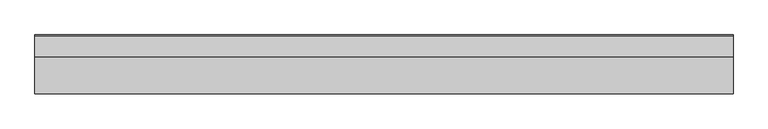
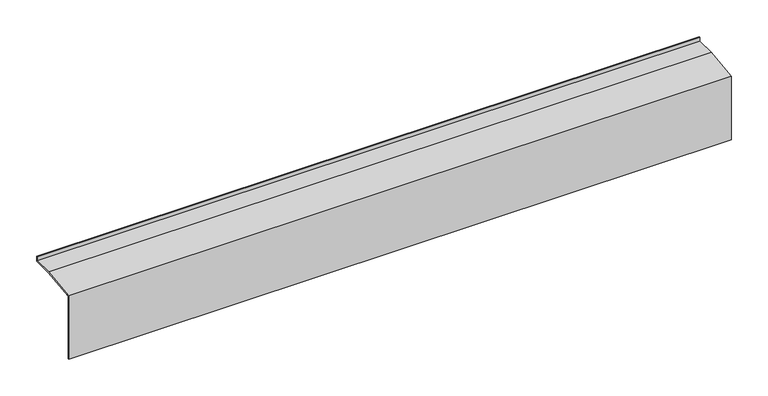
"""IFC4 building model written with IfcOpenShell, lengths in millimetres: proxy geometry, Generic Models 7:Generic Models 1:7:Generic Models 1:7 : Generic Models 7:Generic Models 1:337419:2 : Generic Models 7:Generic Models 1:7:Generic Models 1:7 : Generic Models 7:Generic Models 1:337419:315055."""

from ifc_helpers import new_model, si_unit, frame, origin, place, context, project, spatial, polyline, outline, extrude, source, transform, mapped, element, save


def generic_models_7c3e0f65(model_context):
    return source(origin(), model_context, "Body", "SweptSolid", [
        extrude(outline(polyline([(-579143.2285706, -83.6289841), (-579144.8160706, -83.6289841), (-579144.8160706, 22.420253), (-579089.3872692, 28.575), (-579058.4545584, 28.575), (-579058.4545584, 35.3140132), (-579056.8670584, 35.3140132), (-579056.8670584, 26.9875), (-579089.2994022, 26.9875), (-579143.2285706, 20.9992705), (-579143.2285706, -83.6289841)])), frame((591714.0570845, 0.0, 0.0), z_axis=(1.0, 0.0, 0.0), x_axis=(0.0, 1.0, 0.0)), (0.0, 0.0, 1.0), 1044.8567691),
    ])


if __name__ == "__main__":
    model = new_model("IFC4")
    model_context = context("Model", 3, world=origin())
    ifc_project = project(units=[si_unit("LENGTHUNIT", "METRE", prefix="MILLI")], contexts=[model_context])
    site = spatial("IfcSite", under=ifc_project)
    building = spatial("IfcBuilding", under=site)
    placement = place(None, origin())
    generic_models_shape = generic_models_7c3e0f65(model_context)
    element("IfcBuildingElementProxy", 1, Name="Generic Models 7:Generic Models 1:7:Generic Models 1:7 : Generic Models 7:Generic Models 1:337419:2 : Generic Models 7:Generic Models 1:7:Generic Models 1:7 : Generic Models 7:Generic Models 1:337419:315055", ObjectType="Generic Models 7:Generic Models 1:7:Generic Models 1:7 : Generic Models 7:Generic Models 1:337419:2 : Generic Models 7:Generic Models 1:7:Generic Models 1:7 : Generic Models 7:Generic Models 1:337419:315055", at=placement, inside=building, context=model_context, shape_type="MappedRepresentation", body=[
        mapped(generic_models_shape, transform((0.0, 0.0, 0.0), x_axis=(1.0, 0.0, 0.0), y_axis=(0.0, 1.0, 0.0), z_axis=(0.0, 0.0, 1.0))),
    ])
    save(model, "model.ifc")

# Revit data of these elements
# Type "Generic Models 7:Generic Models 1:7:Generic Models 1:7 : Generic Models 7:Generic Models 1:337419:2 : Generic Models 7:Generic Models 1:7:Generic Models 1:7 : Generic Models 7:Generic Models 1:337419:315055"
#   NameOverride = "Generic Models 7:Generic Models 1:7:Generic Models 1:7 : Generic Models 7:Generic Models 1:337419:315055"
#   ObjectTypeOverride = "Generic Models 1:7 : Generic Models 7:Generic Models 1:337419"
#   Reference = "Generic Models 1"
#   Tag = "315055"
# Element 1 (IfcBuildingElementProxy, "Generic Models 7:Generic Models 1:7:Generic Models 1:7 : Generic Models 7:Generic Models 1:337419:2 : Generic Models 7:Generic Models 1:7:Generic Models 1:7 : Generic Models 7:Generic Models 1:337419:315055")
#   Materials on its faces: "ANODIZED ALUM. FLASHING - MATCH STOREFRONT (ALIGN WITH OTHER WALL ASSEMBLIES)"
# Materials
#   "ANODIZED ALUM. FLASHING - MATCH STOREFRONT (ALIGN WITH OTHER WALL ASSEMBLIES)": class "Unassigned", colour RGB 210 209 208, transparency 0, Cost = 0
